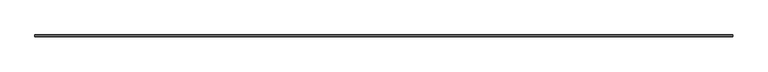
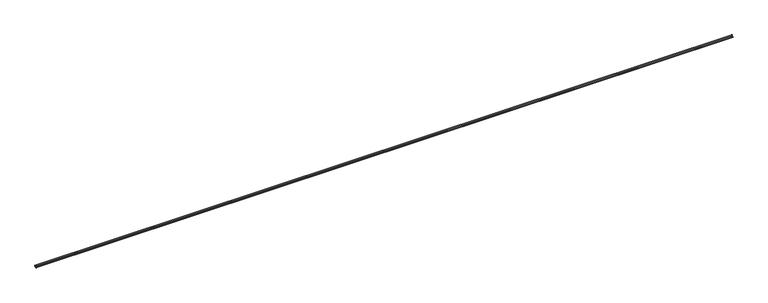
"""IFC4 building model written with IfcOpenShell, lengths in millimetres: proxy geometry, Generic Models 7:Generic Models 1:337419:Generic Models 1:337419 : Generic Models 7:Generic Models 1:337419:9 : Generic Models 7:Generic Models 1:337419:Generic Models 1:337419 : Generic Models 7:Generic Models 1:337419:301336."""

from ifc_helpers import new_model, si_unit, frame, origin, place, context, project, spatial, polyline, outline, extrude, source, transform, mapped, element, save


def generic_models_faac26d3(model_context):
    return source(origin(), model_context, "Body", "SweptSolid", [
        extrude(outline(polyline([(-568228.2483392, 4481.752118), (-568350.3997175, 4476.6624772), (-568365.1162688, 4448.5291231), (-568426.8080098, 4445.9586339), (-568426.7419213, 4444.3725101), (-568417.5044349, 4444.7574054), (-568417.4713906, 4443.9643435), (-568427.501939, 4443.546404), (-568427.6341159, 4446.7186515), (-568365.6071876, 4449.3031068), (-568350.8906362, 4477.436461), (-568229.0420892, 4482.5134838), (-568229.0420892, 4602.402118), (-568228.2483392, 4602.402118), (-568228.2483392, 4481.752118)])), frame((591306.0367242, 0.0, 0.0), z_axis=(1.0, 0.0, 0.0), x_axis=(0.0, 1.0, 0.0)), (0.0, 0.0, 1.0), 76038.0749997),
    ])


if __name__ == "__main__":
    model = new_model("IFC4")
    model_context = context("Model", 3, world=origin())
    ifc_project = project(units=[si_unit("LENGTHUNIT", "METRE", prefix="MILLI")], contexts=[model_context])
    site = spatial("IfcSite", under=ifc_project)
    building = spatial("IfcBuilding", under=site)
    placement = place(None, origin())
    generic_models_shape = generic_models_faac26d3(model_context)
    element("IfcBuildingElementProxy", 1, Name="Generic Models 7:Generic Models 1:337419:Generic Models 1:337419 : Generic Models 7:Generic Models 1:337419:9 : Generic Models 7:Generic Models 1:337419:Generic Models 1:337419 : Generic Models 7:Generic Models 1:337419:301336", ObjectType="Generic Models 7:Generic Models 1:337419:Generic Models 1:337419 : Generic Models 7:Generic Models 1:337419:9 : Generic Models 7:Generic Models 1:337419:Generic Models 1:337419 : Generic Models 7:Generic Models 1:337419:301336", at=placement, inside=building, context=model_context, shape_type="MappedRepresentation", body=[
        mapped(generic_models_shape, transform((0.0, 0.0, 0.0), x_axis=(1.0, 0.0, 0.0), y_axis=(0.0, 1.0, 0.0), z_axis=(0.0, 0.0, 1.0))),
    ])
    save(model, "model.ifc")

# Revit data of these elements
# Type "Generic Models 7:Generic Models 1:337419:Generic Models 1:337419 : Generic Models 7:Generic Models 1:337419:9 : Generic Models 7:Generic Models 1:337419:Generic Models 1:337419 : Generic Models 7:Generic Models 1:337419:301336"
#   NameOverride = "Generic Models 7:Generic Models 1:337419:Generic Models 1:337419 : Generic Models 7:Generic Models 1:337419:301336"
#   ObjectTypeOverride = "Generic Models 1:337419 : Generic Models 7:Generic Models 1:337419"
#   Reference = "Generic Models 1"
#   Tag = "301336"
# Element 1 (IfcBuildingElementProxy, "Generic Models 7:Generic Models 1:337419:Generic Models 1:337419 : Generic Models 7:Generic Models 1:337419:9 : Generic Models 7:Generic Models 1:337419:Generic Models 1:337419 : Generic Models 7:Generic Models 1:337419:301336")
#   Materials on its faces: "PARAPET HIGH EAVE TRIM"
# Materials
#   "PARAPET HIGH EAVE TRIM": class "Unassigned", colour RGB 182 182 182, transparency 0, Cost = 0
